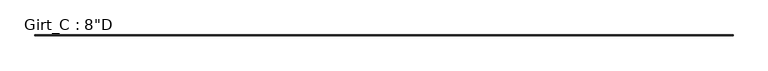
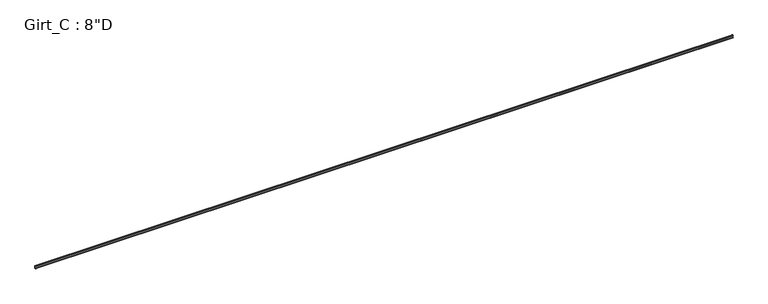
"""IFC4 building model written with IfcOpenShell, lengths in millimetres: beam geometry."""

from ifc_helpers import new_model, si_unit, point, frame, frame_2d, origin, place, context, project, spatial, polyline, circle_curve, trimmed, segment, composite_curve, outline, extrude, source, transform, mapped, element, save


def beam_f72db623(model_context):
    return source(origin(), model_context, "Body", "SweptSolid", [
        extrude(outline(composite_curve([segment(polyline([(-63.5, 101.6), (-3.3734375, 101.6)]), True, "CONTINUOUS"), segment(trimmed(circle_curve(frame_2d((-3.3734375, 96.8375)), 4.7625), [point((-3.3734375, 101.6))], [point((1.3890625, 96.8375))], False, "CARTESIAN"), True, "CONTINUOUS"), segment(polyline([(1.3890625, 96.8375), (1.3890625, -96.8375)]), True, "CONTINUOUS"), segment(trimmed(circle_curve(frame_2d((-3.3734375, -96.8375)), 4.7625), [point((1.3890625, -96.8375))], [point((-3.3734375, -101.6))], False, "CARTESIAN"), True, "CONTINUOUS"), segment(polyline([(-3.3734375, -101.6), (-63.5, -101.6), (-75.745104, -87.0068534), (-73.6169367, -85.221109), (-62.204539, -98.821875), (-3.2694106, -98.821875)]), True, "CONTINUOUS"), segment(trimmed(circle_curve(frame_2d((-3.3748024, -96.8389339)), 1.9857399), [point((-3.2694106, -98.821875))], [point((-1.3890625, -96.8389339))], True, "CARTESIAN"), True, "CONTINUOUS"), segment(polyline([(-1.3890625, -96.8389339), (-1.3890625, 96.8381931)]), True, "CONTINUOUS"), segment(trimmed(circle_curve(frame_2d((-3.3741066, 96.8381931)), 1.9850441), [point((-1.3890625, 96.8381931))], [point((-3.3005807, 98.821875))], True, "CARTESIAN"), True, "CONTINUOUS"), segment(polyline([(-3.3005807, 98.821875), (-62.204539, 98.821875), (-73.6169367, 85.221109), (-75.745104, 87.0068534), (-63.5, 101.6)]), True, "CONTINUOUS")], self_intersect=False)), frame((-26695.4, 0.0, 0.0), z_axis=(1.0, 0.0, 0.0), x_axis=(0.0, 1.0, 0.0)), (0.0, 0.0, 1.0), 53390.8),
    ])


if __name__ == "__main__":
    model = new_model("IFC4")
    model_context = context("Model", 3, world=origin())
    ifc_project = project(units=[si_unit("LENGTHUNIT", "METRE", prefix="MILLI")], contexts=[model_context])
    site = spatial("IfcSite", under=ifc_project)
    building = spatial("IfcBuilding", under=site)
    placement = place(None, origin())
    beam_shape = beam_f72db623(model_context)
    element("IfcBeam", 1, ObjectType="Girt_C : 8\"D", at=placement, inside=building, context=model_context, shape_type="MappedRepresentation", body=[
        mapped(beam_shape, transform((0.0, 0.0, 0.0), x_axis=(1.0, 0.0, 0.0), y_axis=(0.0, 1.0, 0.0), z_axis=(0.0, 0.0, 1.0))),
    ])
    save(model, "model.ifc")

# Revit data of these elements
# Type "Girt_C : 8\"D"
#   Web_Thickness = 0' - 0 7/64"
#   Length [instance default] = 10' - 0"
#   Leg_1 = 0' - 2 1/2"
#   Height = 0' - 8"
#   Structural Material [instance default] = none
# Element 1 (IfcBeam, "Girt_C : 8\"D")
#   Structural Material = Steel
#   Materials on its faces: "Steel"
# Materials
#   "Steel": class "Metal", colour RGB 118 118 114, transparency 0, Description = "Steel, mill finish", Cost = 0
